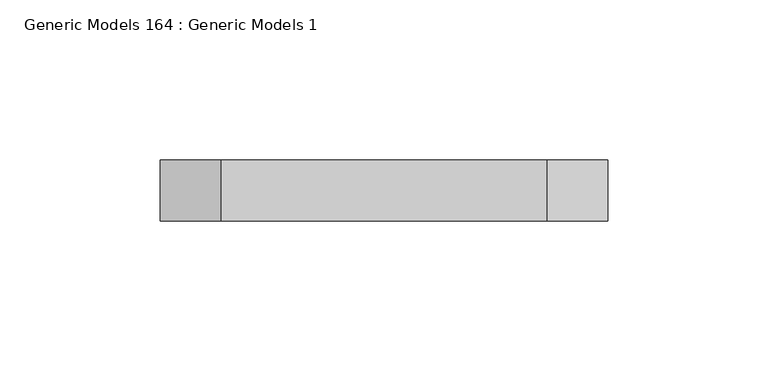
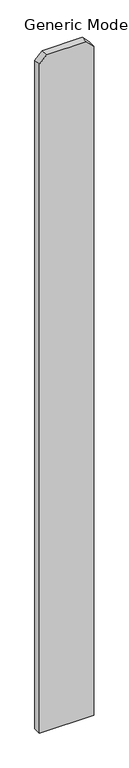
"""IFC4 building model written with IfcOpenShell, lengths in millimetres: proxy geometry, Generic Models 164 : Generic Models 1."""

from ifc_helpers import new_model, si_unit, frame, origin, place, context, project, spatial, polyline, outline, extrude, source, transform, mapped, element, save


def generic_models_164_generic_models_1_488df0f1(model_context):
    return source(origin(), model_context, "Body", "SweptSolid", [
        extrude(outline(polyline([(76.2, -249810.5875), (1885.95, -249810.5875), (1905.0, -249829.6375), (1905.0, -249931.2375), (1885.95, -249950.2875), (76.2, -249950.2875), (76.2, -249810.5875)])), frame((0.0, 547.6875, 0.0), z_axis=(0.0, 1.0, 0.0), x_axis=(0.0, 0.0, 1.0)), (0.0, 0.0, 1.0), 19.05),
    ])


if __name__ == "__main__":
    model = new_model("IFC4")
    model_context = context("Model", 3, world=origin())
    ifc_project = project(units=[si_unit("LENGTHUNIT", "METRE", prefix="MILLI")], contexts=[model_context])
    site = spatial("IfcSite", under=ifc_project)
    building = spatial("IfcBuilding", under=site)
    placement = place(None, origin())
    generic_models_164_generic_models_1_shape = generic_models_164_generic_models_1_488df0f1(model_context)
    element("IfcBuildingElementProxy", 1, Name="Generic Models 164 : Generic Models 1", ObjectType="Generic Models 164 : Generic Models 1", at=placement, inside=building, context=model_context, shape_type="MappedRepresentation", body=[
        mapped(generic_models_164_generic_models_1_shape, transform((0.0, 0.0, 0.0), x_axis=(1.0, 0.0, 0.0), y_axis=(0.0, 1.0, 0.0), z_axis=(0.0, 0.0, 1.0))),
    ])
    save(model, "model.ifc")

# Revit data of these elements
# Element 1 (IfcBuildingElementProxy, "Generic Models 164 : Generic Models 1")
#   Materials on its faces: "VERTICAL 1X6 CEDAR PLANKS W/ CLEAR WOOD SEALER"
# Materials
#   "VERTICAL 1X6 CEDAR PLANKS W/ CLEAR WOOD SEALER": class "Wood", colour RGB 234 198 147, transparency 0, Description = "Pinus Echinata", Cost = 0
